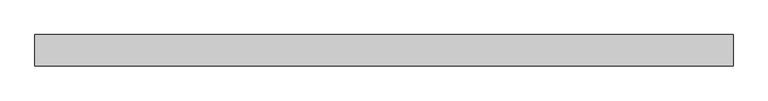
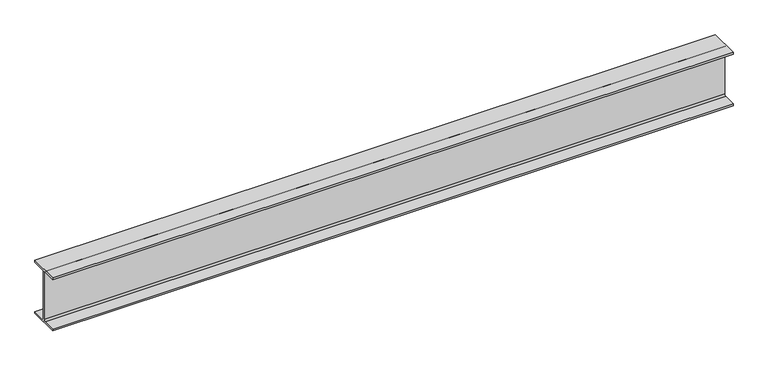
"""IFC4 building model written with IfcOpenShell, lengths in millimetres: beam geometry, Old_Steel Beam_H-KSD3502 : H_SB_ASB_H-340×250x9x14."""

import ifcopenshell
import ifcopenshell.guid

model = None  # the IFC model being written
_history = None  # IfcOwnerHistory: only IFC2X3 demands one
_inside = {}  # id of a spatial element -> (the spatial element, [elements in it])
_under = {}  # id of a project, library or spatial element -> (it, [spatial elements below it])
_declared = {}  # id of a project -> (the project, [libraries it declares])
_typed = {}  # id of a type object -> (the type object, [elements of that type])
_made_of = {}  # id of a material, layer set ... -> (it, [elements and type objects made of it])


def new_model(schema):
    """Start an empty IFC model of exactly this schema.

    Asked for "IFC4X3", IfcOpenShell would pick the latest addendum, in which some entities
    have other attributes; the version numbers below select the first issue.
    IFC2X3 requires an IfcOwnerHistory on every rooted entity: one is made here for all.
    """
    global model, _history
    if schema == "IFC4X3":
        model = ifcopenshell.file(schema_version=(4, 3, 0, 0))
    else:
        model = ifcopenshell.file(schema=schema)
    _inside.clear()
    _under.clear()
    _declared.clear()
    _typed.clear()
    _made_of.clear()
    _history = None
    if model.schema == "IFC2X3":
        org = make("IfcOrganization", Name="unknown")
        user = make(
            "IfcPersonAndOrganization",
            ThePerson=make("IfcPerson", FamilyName="unknown"),
            TheOrganization=org,
        )
        app = make(
            "IfcApplication",
            ApplicationDeveloper=org,
            Version="unknown",
            ApplicationFullName="unknown",
            ApplicationIdentifier="unknown",
        )
        _history = make(
            "IfcOwnerHistory",
            OwningUser=user,
            OwningApplication=app,
            ChangeAction="ADDED",
            CreationDate=0,
        )
    return model


def make(cls, **values):
    """One entity of the class cls with the attributes given. An attribute that is None is left unset."""
    return model.create_entity(
        cls, **{name: value for name, value in values.items() if value is not None}
    )


def rooted(cls, **values):
    """An entity with a GlobalId (a new one), such as an element, a storey or a relation."""
    return make(cls, GlobalId=ifcopenshell.guid.new(), OwnerHistory=_history, **values)


def si_unit(unit_type, name, prefix=None):
    """IfcSIUnit, for example si_unit("LENGTHUNIT", "METRE", prefix="MILLI")."""
    return make("IfcSIUnit", UnitType=unit_type, Prefix=prefix, Name=name)


def assignment(units):
    """IfcUnitAssignment: the units of a project."""
    return None if units is None else make("IfcUnitAssignment", Units=units)


def point(xyz):
    """IfcCartesianPoint."""
    return None if xyz is None else make("IfcCartesianPoint", Coordinates=xyz)


def direction(xyz):
    """IfcDirection."""
    return None if xyz is None else make("IfcDirection", DirectionRatios=xyz)


def frame(location, z_axis=None, x_axis=None):
    """IfcAxis2Placement3D, a coordinate frame: its origin and axes. An axis left out is left unset."""
    return make(
        "IfcAxis2Placement3D",
        Location=point(location),
        Axis=direction(z_axis),
        RefDirection=direction(x_axis),
    )


def frame_2d(location, x_axis=None):
    """IfcAxis2Placement2D, a coordinate frame in the plane: its origin and x axis."""
    return make(
        "IfcAxis2Placement2D", Location=point(location), RefDirection=direction(x_axis)
    )


def origin():
    """The frame at (0, 0, 0) with its axes left unset."""
    return frame((0.0, 0.0, 0.0))


def place(relative_to, where):
    """IfcLocalPlacement: puts the frame where relative to a parent placement (None: the world)."""
    return make(
        "IfcLocalPlacement", PlacementRelTo=relative_to, RelativePlacement=where
    )


def context(
    kind, dimensions, precision=None, world=None, true_north=None, identifier=None
):
    """IfcGeometricRepresentationContext, for example the 3D "Model" context."""
    return make(
        "IfcGeometricRepresentationContext",
        ContextIdentifier=identifier,
        ContextType=kind,
        CoordinateSpaceDimension=dimensions,
        Precision=precision,
        WorldCoordinateSystem=world,
        TrueNorth=true_north,
    )


def project(units=None, contexts=None):
    """IfcProject with its units and contexts."""
    return rooted(
        "IfcProject",
        Name="project",
        RepresentationContexts=contexts,
        UnitsInContext=assignment(units),
    )


def spatial(cls, under=None, at=None, **own):
    """A site, building, storey or space (cls), placed at a placement, below another one or the project."""
    s = rooted(cls, ObjectPlacement=at, **own)
    if under is not None:
        _under.setdefault(under.id(), (under, []))[1].append(s)
    return s


def polyline(points):
    """IfcPolyline through the points."""
    return make("IfcPolyline", Points=[point(p) for p in points])


def circle_curve(where, radius):
    """IfcCircle in the frame where."""
    return make("IfcCircle", Position=where, Radius=radius)


def trimmed(basis, trim1, trim2, sense, master):
    """IfcTrimmedCurve: the piece of a basis curve between two trims."""
    return make(
        "IfcTrimmedCurve",
        BasisCurve=basis,
        Trim1=trim1,
        Trim2=trim2,
        SenseAgreement=sense,
        MasterRepresentation=master,
    )


def segment(curve, same_sense, transition):
    """IfcCompositeCurveSegment."""
    return make(
        "IfcCompositeCurveSegment",
        Transition=transition,
        SameSense=same_sense,
        ParentCurve=curve,
    )


def composite_curve(segments, self_intersect=None):
    """IfcCompositeCurve: segments joined end to end."""
    return make("IfcCompositeCurve", Segments=segments, SelfIntersect=self_intersect)


def outline(outer, holes=None, kind="AREA"):
    """IfcArbitraryClosedProfileDef: a profile drawn as a closed curve; with holes, ...WithVoids."""
    if holes is None:
        return make("IfcArbitraryClosedProfileDef", ProfileType=kind, OuterCurve=outer)
    return make(
        "IfcArbitraryProfileDefWithVoids",
        ProfileType=kind,
        OuterCurve=outer,
        InnerCurves=holes,
    )


def extrude(swept, where, along, depth):
    """IfcExtrudedAreaSolid: the profile swept, set in the frame where, extruded along a direction by depth."""
    return make(
        "IfcExtrudedAreaSolid",
        SweptArea=swept,
        Position=where,
        ExtrudedDirection=direction(along),
        Depth=depth,
    )


def shape(context_of_items, identifier, shape_type, items):
    """IfcShapeRepresentation: the items that make up one representation, for example the "Body"."""
    return make(
        "IfcShapeRepresentation",
        ContextOfItems=context_of_items,
        RepresentationIdentifier=identifier,
        RepresentationType=shape_type,
        Items=items,
    )


def source(mapping_origin, context_of_items, identifier, shape_type, items):
    """IfcRepresentationMap: a shape defined once, which mapped items show again and again."""
    return make(
        "IfcRepresentationMap",
        MappingOrigin=mapping_origin,
        MappedRepresentation=shape(context_of_items, identifier, shape_type, items),
    )


def transform(
    local_origin,
    x_axis=None,
    y_axis=None,
    z_axis=None,
    scale=None,
    scale2=None,
    scale3=None,
    uniform=True,
):
    """IfcCartesianTransformationOperator3D, or its non-uniform kind. x_axis, y_axis, z_axis: its Axis1, 2, 3."""
    if uniform:
        return make(
            "IfcCartesianTransformationOperator3D",
            Axis1=direction(x_axis),
            Axis2=direction(y_axis),
            LocalOrigin=point(local_origin),
            Scale=scale,
            Axis3=direction(z_axis),
        )
    return make(
        "IfcCartesianTransformationOperator3DnonUniform",
        Axis1=direction(x_axis),
        Axis2=direction(y_axis),
        LocalOrigin=point(local_origin),
        Scale=scale,
        Axis3=direction(z_axis),
        Scale2=scale2,
        Scale3=scale3,
    )


def mapped(mapping_source, mapping_target):
    """IfcMappedItem: shows the shape of a source again, moved by a transform."""
    return make(
        "IfcMappedItem", MappingSource=mapping_source, MappingTarget=mapping_target
    )


def made_of(thing, what):
    """Note that an element or type object is made of a material, layer set ...; save() writes the relation."""
    if what is not None:
        _made_of.setdefault(what.id(), (what, []))[1].append(thing)
    return thing


def element(
    cls,
    number,
    at=None,
    inside=None,
    cuts=None,
    type_object=None,
    material=None,
    context=None,
    identifier="Body",
    shape_type=None,
    held_by="IfcProductDefinitionShape",
    body=None,
    shapes=None,
    **own,
):
    """One element of the class cls, such as IfcWall. Its Tag is "e" and its number.

    at: its placement. inside: the storey or other place that contains it. cuts: it is an
    opening in that element (IfcRelVoidsElement). A single representation is given by context,
    identifier, shape_type and body (its items); several are given by shapes. held_by: the class
    of the entity that holds the representations. save() writes the other relations.
    """
    e = rooted(cls, Tag="e%d" % number, ObjectPlacement=at, **own)
    if body is not None:
        shapes = [shape(context, identifier, shape_type, body)]
    if shapes is not None:
        e.Representation = make(held_by, Representations=shapes)
    if inside is not None:
        _inside.setdefault(inside.id(), (inside, []))[1].append(e)
    if cuts is not None:
        rooted(
            "IfcRelVoidsElement", RelatingBuildingElement=cuts, RelatedOpeningElement=e
        )
    if type_object is not None:
        _typed.setdefault(type_object.id(), (type_object, []))[1].append(e)
    return made_of(e, material)


def aggregate(whole, parts):
    """IfcRelAggregates: a whole, such as a stair, and the parts it consists of."""
    return rooted("IfcRelAggregates", RelatingObject=whole, RelatedObjects=parts)


def save(model, path):
    """Write the relations noted so far, then the file.

    IfcRelAggregates (storeys below a building ...), IfcRelContainedInSpatialStructure (elements
    in a storey), IfcRelDefinesByType, IfcRelAssociatesMaterial and IfcRelDeclares: one each for
    every whole, place, type object, material and project.
    """
    for whole, parts in _under.values():
        aggregate(whole, parts)
    for where, things in _inside.values():
        rooted(
            "IfcRelContainedInSpatialStructure",
            RelatedElements=things,
            RelatingStructure=where,
        )
    for kind, things in _typed.values():
        rooted("IfcRelDefinesByType", RelatedObjects=things, RelatingType=kind)
    for what, things in _made_of.values():
        rooted("IfcRelAssociatesMaterial", RelatedObjects=things, RelatingMaterial=what)
    for by, libraries in _declared.values():
        rooted("IfcRelDeclares", RelatingContext=by, RelatedDefinitions=libraries)
    model.write(path)


def beam_4818db7e(model_context):
    return source(origin(), model_context, "Body", "SweptSolid", [
        extrude(outline(composite_curve([segment(polyline([(82.5, -141.5), (82.5, -151.7), (-82.5, -151.7), (-82.5, -141.5), (-11.9, -141.5)]), True, "CONTINUOUS"), segment(trimmed(circle_curve(frame_2d((-11.9, -132.6)), 8.9), [point((-11.9, -141.5))], [point((-3.0, -132.6))], True, "CARTESIAN"), True, "CONTINUOUS"), segment(polyline([(-3.0, -132.6), (-3.0, 132.6)]), True, "CONTINUOUS"), segment(trimmed(circle_curve(frame_2d((-11.9, 132.6)), 8.9), [point((-3.0, 132.6))], [point((-11.9, 141.5))], True, "CARTESIAN"), True, "CONTINUOUS"), segment(polyline([(-11.9, 141.5), (-82.5, 141.5), (-82.5, 151.7), (82.5, 151.7), (82.5, 141.5), (11.9, 141.5)]), True, "CONTINUOUS"), segment(trimmed(circle_curve(frame_2d((11.9, 132.6)), 8.9), [point((11.9, 141.5))], [point((3.0, 132.6))], True, "CARTESIAN"), True, "CONTINUOUS"), segment(polyline([(3.0, 132.6), (3.0, -132.6)]), True, "CONTINUOUS"), segment(trimmed(circle_curve(frame_2d((11.9, -132.6)), 8.9), [point((3.0, -132.6))], [point((11.9, -141.5))], True, "CARTESIAN"), True, "CONTINUOUS"), segment(polyline([(11.9, -141.5), (82.5, -141.5)]), True, "CONTINUOUS")], self_intersect=False)), frame((-1837.3, 0.0, 0.0), z_axis=(1.0, 0.0, 0.0), x_axis=(0.0, 1.0, 0.0)), (0.0, 0.0, 1.0), 3674.6),
    ])


if __name__ == "__main__":
    model = new_model("IFC4")
    model_context = context("Model", 3, world=origin())
    ifc_project = project(units=[si_unit("LENGTHUNIT", "METRE", prefix="MILLI")], contexts=[model_context])
    site = spatial("IfcSite", under=ifc_project)
    building = spatial("IfcBuilding", under=site)
    placement = place(None, origin())
    beam_shape = beam_4818db7e(model_context)
    element("IfcBeam", 1, ObjectType="Old_Steel Beam_H-KSD3502 : H_SB_ASB_H-340×250x9x14", at=placement, inside=building, context=model_context, shape_type="MappedRepresentation", body=[
        mapped(beam_shape, transform((0.0, 0.0, 0.0), x_axis=(1.0, 0.0, 0.0), y_axis=(0.0, 1.0, 0.0), z_axis=(0.0, 0.0, 1.0))),
    ])
    save(model, "model.ifc")

# Revit data of these elements
# Type "Old_Steel Beam_H-KSD3502 : H_SB_ASB_H-340×250x9x14"
#   Width = 25.0 cm
#   Web Thickness = 0.9 cm
#   Web Fillet = 2.0 cm
#   Warping Constant = 968661.0 cm⁶
#   Torsional Moment of Inertia = 53.6551 cm⁴
#   Torsional Modulus = 1.0 cm³
#   Section Area = 101.5 cm²
#   Plastic Modulus weak axis = 447.0 cm³
#   Plastic Modulus strong axis = 1410.0 cm³
#   Perimeter = 1.63 m²/m
#   Nominal Weight = 79.70 kgf/m
#   Moment of Inertia weak axis = 3650.00 cm⁴
#   Moment of Inertia strong axis = 21700.00 cm⁴
#   Height = 34.0 cm
#   Flange Thickness = 1.4 cm
#   Elastic Modulus weak axis = 292.0 cm³
#   Elastic Modulus strong axis = 1280.0 cm³
#   Centroid Vertical = 17.0 cm
#   Centroid Horizontal = 12.5 cm
#   Length [instance default] = 1.5240 m
#   Structural Material [instance default] = Steel, 45-345
#   Assembly Code = ""
# Element 1 (IfcBeam, "Old_Steel Beam_H-KSD3502 : H_SB_ASB_H-340×250x9x14")
#   Structural Material = none
# Materials
#   "Steel, 45-345": class "Metal", colour RGB 189 187 185, transparency 0, Description = "Steel 345 MPa", Cost = 0
